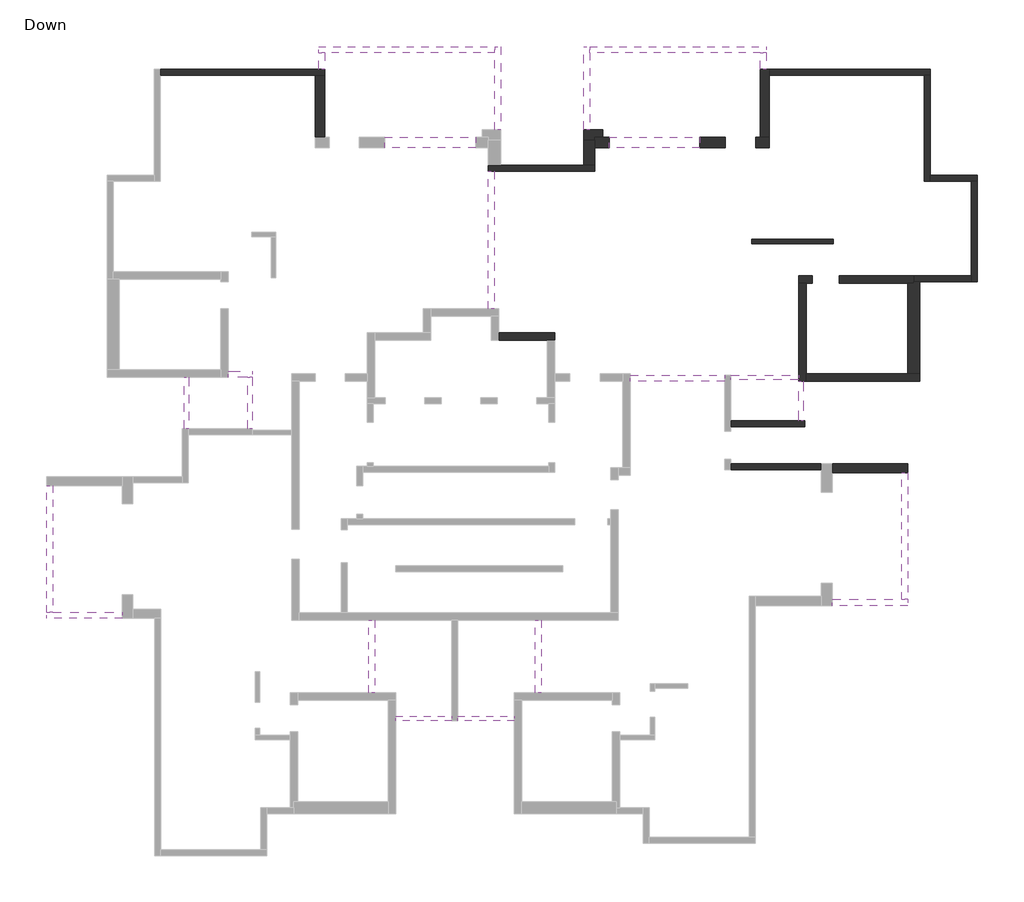
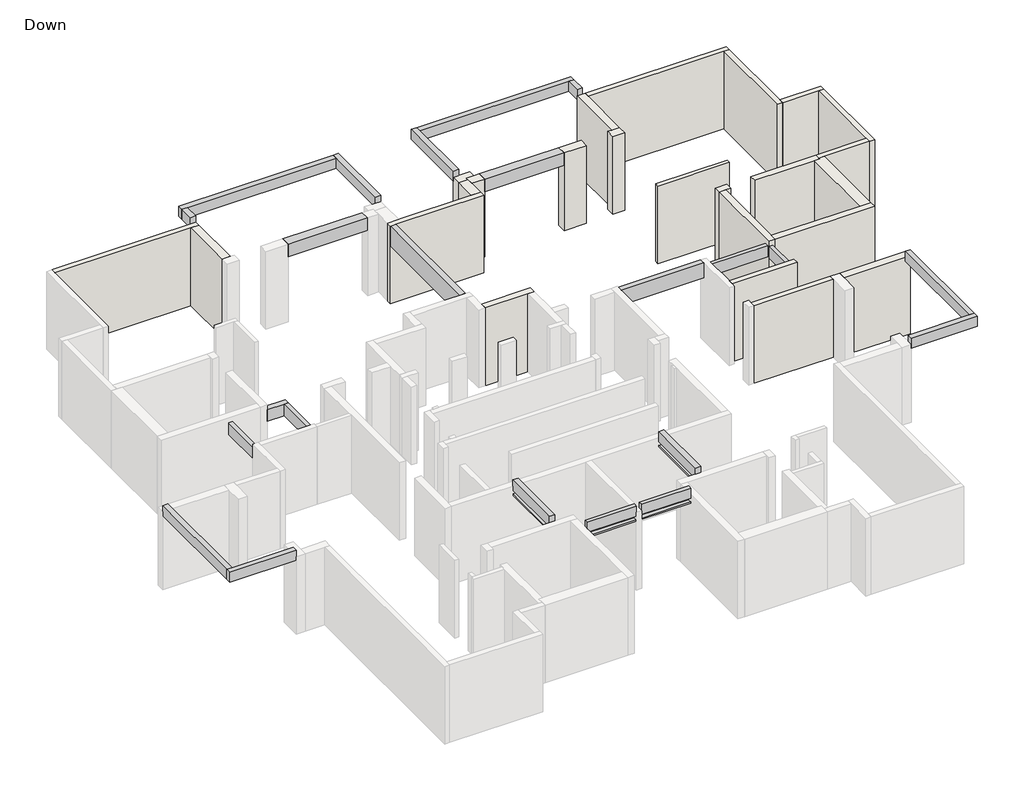
# One storey, part 3 of 3: 24 walls, 23 beams.
"""IFC4 building model written with IfcOpenShell, lengths in millimetres."""

from ifc_helpers import new_model, si_unit, frame, origin, place, context, project, spatial, polyline, outline, extrude, faceted_brep, element, save

model = new_model("IFC4")

# Units and contexts
model_context = context("Model", 3, world=origin())
ifc_project = project(units=[si_unit("LENGTHUNIT", "METRE", prefix="MILLI")], contexts=[model_context])

# Site, building, storey
site = spatial("IfcSite", under=ifc_project)
building = spatial("IfcBuilding", under=site)
storey = spatial("IfcBuildingStorey", under=building, Name="Down", Elevation=0.0)

# Beams
placement = place(None, origin())
element("IfcBeam", 1, ObjectType="Concrete Rectengular Beam : 15/60", at=placement, inside=storey, context=model_context, shape_type="Brep", body=[
    faceted_brep([(26027.850174, -8804.7310591, 2900.0), (26027.850174, -8954.7310591, 2900.0), (26027.850174, -8954.7310591, 2450.0), (26027.850174, -8804.7310591, 2450.0), (26027.850174, -8804.7310591, 2730.0), (23780.6220263, -8954.7310591, 2900.0), (23780.6220263, -8804.7310591, 2900.0), (23780.6220263, -8804.7310591, 2450.0), (23780.6220263, -8954.7310591, 2450.0)], [[[0, 1, 2, 3, 4]], [[5, 6, 7, 8]], [[1, 0, 6, 5]], [[1, 5, 8, 2]], [[6, 0, 4, 3, 7]], [[3, 2, 8, 7]]]),
])
element("IfcBeam", 2, ObjectType="Concrete Rectengular Beam : 15/60", at=placement, inside=storey, context=model_context, shape_type="SweptSolid", body=[
    extrude(outline(polyline([(26177.850174, -10305.7627314), (26027.850174, -10305.7627314), (26027.850174, -9003.4933914), (26177.850174, -9003.4933914), (26177.850174, -10305.7627314)])), frame((0.0, 0.0, 2450.0), z_axis=(0.0, 0.0, 1.0), x_axis=(1.0, 0.0, 0.0)), (0.0, 0.0, 1.0), 450.0),
])
element("IfcBeam", 3, ObjectType="Concrete Rectengular Beam : 15/60", at=placement, inside=storey, context=model_context, shape_type="SweptSolid", body=[
    extrude(outline(polyline([(5696.9503171, -8875.9821525), (5846.9503171, -8875.9821525), (5846.9503171, -10574.5447275), (5696.9503171, -10574.5447275), (5696.9503171, -8875.9821525)])), frame((0.0, 0.0, 2450.0), z_axis=(0.0, 0.0, 1.0), x_axis=(1.0, 0.0, 0.0)), (0.0, 0.0, 1.0), 450.0),
])
element("IfcBeam", 4, ObjectType="Concrete Rectengular Beam : 15/60", at=placement, inside=storey, context=model_context, shape_type="Brep", body=[
    faceted_brep([(7954.0579731, -10574.5447275, 2900.0), (7804.0579731, -10574.5447275, 2900.0), (7804.0579731, -10574.5447275, 2450.0), (7954.0579731, -10574.5447275, 2450.0), (7954.0579731, -10574.5447275, 2730.0), (7954.0579731, -8873.5161743, 2900.0), (7804.0579731, -8873.5161743, 2900.0), (7804.0579731, -8873.5161743, 2450.0), (7954.0579731, -8873.5161743, 2450.0), (7954.0579731, -8873.5161743, 2730.0)], [[[0, 1, 2, 3, 4]], [[1, 0, 5, 6]], [[1, 6, 7, 2]], [[5, 0, 4, 3, 8, 9]], [[6, 5, 9, 8, 7]], [[3, 2, 7, 8]]]),
])
element("IfcBeam", 5, ObjectType="Concrete Rectengular Beam : 15/60", at=placement, inside=storey, context=model_context, shape_type="Brep", body=[
    faceted_brep([(14556.9532328, -20224.3060494, 2750.0), (14556.9532328, -20074.3060494, 2750.0), (14556.9532328, -20074.3060494, 2800.0), (14556.9532328, -20224.3060494, 2800.0), (12702.1320718, -20074.3060494, 2750.0), (12702.1320718, -20224.3060494, 2750.0), (12702.1320718, -20224.3060494, 2800.0), (12702.1320718, -20074.3060494, 2800.0)], [[[0, 1, 2, 3]], [[4, 5, 6, 7]], [[1, 0, 5, 4]], [[1, 4, 7, 2]], [[3, 2, 7, 6]], [[5, 0, 3, 6]]]),
    faceted_brep([(14556.9532328, -20224.3060494, 3350.0), (14556.9532328, -20074.3060494, 3350.0), (12702.1320718, -20074.3060494, 3350.0), (12702.1320718, -20224.3060494, 3350.0), (12702.1320718, -20224.3060494, 2950.0), (14556.9532328, -20224.3060494, 2950.0), (14556.9532328, -20224.3060494, 3100.0), (14556.9532328, -20074.3060494, 2950.0), (12702.1320718, -20074.3060494, 2950.0)], [[[0, 1, 2, 3]], [[0, 3, 4, 5, 6]], [[7, 5, 4, 8]], [[1, 0, 6, 5, 7]], [[3, 2, 8, 4]], [[2, 1, 7, 8]]]),
])
element("IfcBeam", 6, ObjectType="Concrete Rectengular Beam : 15/60", at=placement, inside=storey, context=model_context, shape_type="Brep", body=[
    faceted_brep([(16611.7743938, -20224.3060494, 2750.0), (16611.7743938, -20074.3060494, 2750.0), (16611.7743938, -20074.3060494, 2800.0), (16611.7743938, -20224.3060494, 2800.0), (14756.9532328, -20074.3060494, 2750.0), (14756.9532328, -20224.3060494, 2750.0), (14756.9532328, -20224.3060494, 2800.0), (14756.9532328, -20074.3060494, 2800.0)], [[[0, 1, 2, 3]], [[4, 5, 6, 7]], [[1, 0, 5, 4]], [[1, 4, 7, 2]], [[3, 2, 7, 6]], [[5, 0, 3, 6]]]),
    faceted_brep([(16611.7743938, -20224.3060494, 3350.0), (16611.7743938, -20074.3060494, 3350.0), (14756.9532328, -20074.3060494, 3350.0), (14756.9532328, -20224.3060494, 3350.0), (14756.9532328, -20224.3060494, 3100.0), (14756.9532328, -20224.3060494, 2950.0), (16611.7743938, -20224.3060494, 2950.0), (16611.7743938, -20074.3060494, 2950.0), (14756.9532328, -20074.3060494, 2950.0)], [[[0, 1, 2, 3]], [[0, 3, 4, 5, 6]], [[7, 6, 5, 8]], [[1, 0, 6, 7]], [[3, 2, 8, 5, 4]], [[2, 1, 7, 8]]]),
])
element("IfcBeam", 7, ObjectType="Concrete Rectengular Beam : 20/60", at=placement, inside=storey, context=model_context, shape_type="Brep", body=[
    faceted_brep([(20461.0939579, -8804.7310591, 3100.0), (20461.0939579, -9004.7310591, 3100.0), (23580.6220263, -9004.7310591, 3100.0), (23580.6220263, -8804.7310591, 3100.0), (20461.0939579, -8804.7310591, 2500.0), (20461.0939579, -8804.7310591, 2730.0), (20461.0939579, -8804.7310591, 2950.0), (23580.6220263, -8804.7310591, 2500.0), (20461.0939579, -9004.7310591, 2500.0), (23580.6220263, -9004.7310591, 2500.0), (20461.0939579, -9004.7310591, 2950.0), (20461.0939579, -9004.7310591, 2730.0), (23580.6220263, -9004.7310591, 2730.0), (23580.6220263, -9004.7310591, 2950.0)], [[[0, 1, 2, 3]], [[4, 5, 6, 0, 3, 7]], [[8, 4, 7, 9]], [[1, 10, 11, 8, 9, 12, 13, 2]], [[1, 0, 6, 5, 4, 8, 11, 10]], [[3, 2, 13, 12, 9, 7]]]),
])
element("IfcBeam", 8, ObjectType="Concrete Rectengular Beam : 20/60", at=placement, inside=storey, context=model_context, shape_type="Brep", body=[
    faceted_brep([(16172.9774125, -685.8100602, 3350.0), (15972.9774125, -685.8100602, 3350.0), (15972.9774125, -685.8100602, 2950.0), (16172.9774125, -685.8100602, 2950.0), (16172.9774125, -685.8100602, 3100.0), (16172.9774125, 2066.3547226, 3350.0), (15972.9774125, 2066.3547226, 3350.0), (15972.9774125, 1866.3547226, 3350.0), (16172.9774125, 2066.3547226, 2950.0), (15972.9774125, 2066.3547226, 2950.0), (15972.9774125, 1866.3547226, 2950.0)], [[[0, 1, 2, 3, 4]], [[1, 0, 5, 6, 7]], [[5, 0, 4, 3, 8]], [[1, 7, 6, 9, 10, 2]], [[6, 5, 8, 9]], [[3, 2, 10, 9, 8]]]),
])
element("IfcBeam", 9, ObjectType="Concrete Rectengular Beam : 20/60", at=placement, inside=storey, context=model_context, shape_type="Brep", body=[
    faceted_brep([(10145.0259753, 2066.3547226, 3350.0), (10145.0259753, 1866.3547226, 3350.0), (10345.0259753, 1866.3547226, 3350.0), (15972.9774125, 1866.3547226, 3350.0), (15972.9774125, 2066.3547226, 3350.0), (15972.9774125, 2066.3547226, 2950.0), (10145.0259753, 2066.3547226, 2950.0), (10145.0259753, 1866.3547226, 2950.0), (10345.0259753, 1866.3547226, 2950.0), (15972.9774125, 1866.3547226, 2950.0)], [[[0, 1, 2, 3, 4]], [[0, 4, 5, 6]], [[3, 2, 1, 7, 8, 9]], [[1, 0, 6, 7]], [[4, 3, 9, 5]], [[6, 5, 9, 8, 7]]]),
])
element("IfcBeam", 10, ObjectType="Concrete Rectengular Beam : 20/60", at=placement, inside=storey, context=model_context, shape_type="Brep", body=[
    faceted_brep([(10345.0259753, 1316.3547226, 3350.0), (10145.0259753, 1316.3547226, 3350.0), (10145.0259753, 1316.3547226, 2950.0), (10345.0259753, 1316.3547226, 2950.0), (10345.0259753, 1316.3547226, 3100.0), (10345.0259753, 1866.3547226, 3350.0), (10145.0259753, 1866.3547226, 3350.0), (10145.0259753, 1866.3547226, 2950.0), (10345.0259753, 1866.3547226, 2950.0)], [[[0, 1, 2, 3, 4]], [[1, 0, 5, 6]], [[1, 6, 7, 2]], [[5, 0, 4, 3, 8]], [[6, 5, 8, 7]], [[3, 2, 7, 8]]]),
])
element("IfcBeam", 11, ObjectType="Concrete Rectengular Beam : 20/60", at=placement, inside=storey, context=model_context, shape_type="Brep", body=[
    faceted_brep([(19122.5763384, -685.8100602, 3350.0), (18922.5763384, -685.8100602, 3350.0), (18922.5763384, -685.8100602, 3100.0), (18922.5763384, -685.8100602, 2950.0), (19122.5763384, -685.8100602, 2950.0), (19122.5763384, 1866.3547226, 3350.0), (19122.5763384, 2066.3547226, 3350.0), (18922.5763384, 2066.3547226, 3350.0), (19122.5763384, 1866.3547226, 2950.0), (19122.5763384, 2066.3547226, 2950.0), (18922.5763384, 2066.3547226, 2950.0)], [[[0, 1, 2, 3, 4]], [[1, 0, 5, 6, 7]], [[6, 5, 0, 4, 8, 9]], [[1, 7, 10, 3, 2]], [[7, 6, 9, 10]], [[4, 3, 10, 9, 8]]]),
])
element("IfcBeam", 12, ObjectType="Concrete Rectengular Beam : 20/60", at=placement, inside=storey, context=model_context, shape_type="Brep", body=[
    faceted_brep([(24949.2058247, 1866.3547226, 3350.0), (24949.2058247, 2066.3547226, 3350.0), (19122.5763384, 2066.3547226, 3350.0), (19122.5763384, 1866.3547226, 3350.0), (24749.2058247, 1866.3547226, 3350.0), (19122.5763384, 1866.3547226, 2950.0), (24749.2058247, 1866.3547226, 2950.0), (24949.2058247, 1866.3547226, 2950.0), (24949.2058247, 2066.3547226, 2950.0), (19122.5763384, 2066.3547226, 2950.0)], [[[0, 1, 2, 3, 4]], [[0, 4, 3, 5, 6, 7]], [[2, 1, 8, 9]], [[1, 0, 7, 8]], [[3, 2, 9, 5]], [[7, 6, 5, 9, 8]]]),
])
element("IfcBeam", 13, ObjectType="Concrete Rectengular Beam : 20/60", at=placement, inside=storey, context=model_context, shape_type="Brep", body=[
    faceted_brep([(24949.2058247, 1316.3547226, 3350.0), (24749.2058247, 1316.3547226, 3350.0), (24749.2058247, 1316.3547226, 3100.0), (24749.2058247, 1316.3547226, 2950.0), (24949.2058247, 1316.3547226, 2950.0), (24949.2058247, 1866.3547226, 3350.0), (24749.2058247, 1866.3547226, 3350.0), (24749.2058247, 1866.3547226, 2950.0), (24949.2058247, 1866.3547226, 2950.0)], [[[0, 1, 2, 3, 4]], [[1, 0, 5, 6]], [[1, 6, 7, 3, 2]], [[5, 0, 4, 8]], [[6, 5, 8, 7]], [[4, 3, 7, 8]]]),
])
element("IfcBeam", 14, ObjectType="Concrete Rectengular Beam : 20/60", at=placement, inside=storey, context=model_context, shape_type="Brep", body=[
    faceted_brep([(3654.7368494, -16642.3482114, 3350.0), (3654.7368494, -16842.3482114, 3350.0), (3654.7368494, -16842.3482114, 3100.0), (3654.7368494, -16842.3482114, 2950.0), (3654.7368494, -16642.3482114, 2950.0), (1351.3421966, -16642.3482114, 3350.0), (1151.3421966, -16642.3482114, 3350.0), (1151.3421966, -16842.3482114, 3350.0), (1351.3421966, -16642.3482114, 2950.0), (1151.3421966, -16642.3482114, 2950.0), (1151.3421966, -16842.3482114, 2950.0)], [[[0, 1, 2, 3, 4]], [[1, 0, 5, 6, 7]], [[6, 5, 0, 4, 8, 9]], [[1, 7, 10, 3, 2]], [[7, 6, 9, 10]], [[4, 3, 10, 9, 8]]]),
])
element("IfcBeam", 15, ObjectType="Concrete Rectengular Beam : 20/60", at=placement, inside=storey, context=model_context, shape_type="Brep", body=[
    faceted_brep([(1151.3421966, -12453.0033555, 3350.0), (1351.3421966, -12453.0033555, 3350.0), (1351.3421966, -12453.0033555, 2950.0), (1151.3421966, -12453.0033555, 2950.0), (1151.3421966, -12453.0033555, 3100.0), (1151.3421966, -16642.3482114, 3350.0), (1351.3421966, -16642.3482114, 3350.0), (1351.3421966, -16642.3482114, 2950.0), (1151.3421966, -16642.3482114, 2950.0)], [[[0, 1, 2, 3, 4]], [[1, 0, 5, 6]], [[1, 6, 7, 2]], [[5, 0, 4, 3, 8]], [[6, 5, 8, 7]], [[3, 2, 7, 8]]]),
])
element("IfcBeam", 16, ObjectType="Concrete Rectengular Beam : 20/60", at=placement, inside=storey, context=model_context, shape_type="Brep", body=[
    faceted_brep([(27127.656655, -16418.7263398, 3350.0), (27127.656655, -16218.7263398, 3350.0), (27127.656655, -16218.7263398, 2950.0), (27127.656655, -16418.7263398, 2950.0), (27127.656655, -16418.7263398, 3100.0), (29629.9103996, -16418.7263398, 3350.0), (29629.9103996, -16218.7263398, 3350.0), (29429.9103996, -16218.7263398, 3350.0), (29629.9103996, -16418.7263398, 2950.0), (29629.9103996, -16218.7263398, 2950.0), (29429.9103996, -16218.7263398, 2950.0)], [[[0, 1, 2, 3, 4]], [[1, 0, 5, 6, 7]], [[5, 0, 4, 3, 8]], [[1, 7, 6, 9, 10, 2]], [[6, 5, 8, 9]], [[3, 2, 10, 9, 8]]]),
])
element("IfcBeam", 17, ObjectType="Concrete Rectengular Beam : 20/60", at=placement, inside=storey, context=model_context, shape_type="SweptSolid", body=[
    extrude(outline(polyline([(29429.9103996, -12033.0804512), (29629.9103996, -12033.0804512), (29629.9103996, -16218.7263398), (29429.9103996, -16218.7263398), (29429.9103996, -12033.0804512)])), frame((0.0, 0.0, 2950.0), z_axis=(0.0, 0.0, 1.0), x_axis=(1.0, 0.0, 0.0)), (0.0, 0.0, 1.0), 400.0),
])
element("IfcBeam", 18, ObjectType="Concrete Rectengular Beam : 20/60", at=placement, inside=storey, context=model_context, shape_type="Brep", body=[
    faceted_brep([(7157.9504595, -8873.5161743, 2900.0), (7157.9504595, -8673.5161743, 2900.0), (7157.9504595, -8673.5161743, 2730.0), (7157.9504595, -8673.5161743, 2450.0), (7157.9504595, -8873.5161743, 2450.0), (7804.0579731, -8873.5161743, 2900.0), (7954.0579731, -8873.5161743, 2900.0), (7954.0579731, -8673.5161743, 2900.0), (7804.0579731, -8873.5161743, 2450.0), (7954.0579731, -8873.5161743, 2450.0), (7954.0579731, -8873.5161743, 2730.0), (7954.0579731, -8673.5161743, 2730.0), (7954.0579731, -8673.5161743, 2450.0)], [[[0, 1, 2, 3, 4]], [[1, 0, 5, 6, 7]], [[6, 5, 0, 4, 8, 9, 10]], [[1, 7, 11, 12, 3, 2]], [[7, 6, 10, 9, 12, 11]], [[4, 3, 12, 9, 8]]]),
])
element("IfcBeam", 19, ObjectType="Concrete Rectengular Beam : 20/60", at=placement, inside=storey, context=model_context, shape_type="SweptSolid", body=[
    extrude(outline(polyline([(11800.0437745, -16906.0156488), (12000.0437745, -16906.0156488), (12000.0437745, -19301.9218456), (11800.0437745, -19301.9218456), (11800.0437745, -16906.0156488)])), frame((0.0, 0.0, 2750.0), z_axis=(0.0, 0.0, 1.0), x_axis=(1.0, 0.0, 0.0)), (0.0, 0.0, 1.0), 50.0),
    extrude(outline(polyline([(11800.0437745, -16906.0156488), (12000.0437745, -16906.0156488), (12000.0437745, -19301.9218456), (11800.0437745, -19301.9218456), (11800.0437745, -16906.0156488)])), frame((0.0, 0.0, 2950.0), z_axis=(0.0, 0.0, 1.0), x_axis=(1.0, 0.0, 0.0)), (0.0, 0.0, 1.0), 400.0),
])
element("IfcBeam", 20, ObjectType="Concrete Rectengular Beam : 20/60", at=placement, inside=storey, context=model_context, shape_type="SweptSolid", body=[
    extrude(outline(polyline([(17308.6310988, -16906.0156488), (17508.6310988, -16906.0156488), (17508.6310988, -19301.9218456), (17308.6310988, -19301.9218456), (17308.6310988, -16906.0156488)])), frame((0.0, 0.0, 2750.0), z_axis=(0.0, 0.0, 1.0), x_axis=(1.0, 0.0, 0.0)), (0.0, 0.0, 1.0), 50.0),
    extrude(outline(polyline([(17308.6310988, -16906.0156488), (17508.6310988, -16906.0156488), (17508.6310988, -19301.9218456), (17308.6310988, -19301.9218456), (17308.6310988, -16906.0156488)])), frame((0.0, 0.0, 2950.0), z_axis=(0.0, 0.0, 1.0), x_axis=(1.0, 0.0, 0.0)), (0.0, 0.0, 1.0), 400.0),
])
element("IfcBeam", 21, ObjectType="Concrete Rectengular Beam : 20/80", at=placement, inside=storey, context=model_context, shape_type="Brep", body=[
    faceted_brep([(15755.4299651, -6603.7071845, 3100.0), (15955.4299651, -6603.7071845, 3100.0), (15955.4299651, -2061.9790741, 3100.0), (15755.4299651, -2061.9790741, 3100.0), (15955.4299651, -6603.7071845, 2950.0), (15955.4299651, -6603.7071845, 2730.0), (15955.4299651, -6603.7071845, 2300.0), (15955.4299651, -2061.9790741, 2300.0), (15955.4299651, -2061.9790741, 2730.0), (15955.4299651, -2061.9790741, 2950.0), (15755.4299651, -6603.7071845, 2300.0), (15755.4299651, -2061.9790741, 2300.0), (15755.4299651, -6603.7071845, 2730.0), (15755.4299651, -6603.7071845, 2950.0), (15755.4299651, -2061.9790741, 2950.0), (15755.4299651, -2061.9790741, 2730.0)], [[[0, 1, 2, 3]], [[1, 4, 5, 6, 7, 8, 9, 2]], [[6, 10, 11, 7]], [[10, 12, 13, 0, 3, 14, 15, 11]], [[1, 0, 13, 12, 10, 6, 5, 4]], [[3, 2, 9, 8, 7, 11, 15, 14]]]),
])
element("IfcBeam", 22, ObjectType="Concrete Rectengular Beam : 35/50", at=placement, inside=storey, context=model_context, shape_type="Brep", body=[
    faceted_brep([(12338.469313, -935.8943434, 3100.0), (12338.469313, -1285.8943434, 3100.0), (15339.3043472, -1285.8943434, 3100.0), (15339.3043472, -935.8943434, 3100.0), (12338.469313, -1285.8943434, 2950.0), (12338.469313, -1285.8943434, 2730.0), (12338.469313, -1285.8943434, 2600.0), (15339.3043472, -1285.8943434, 2600.0), (15339.3043472, -1285.8943434, 2730.0), (15339.3043472, -1285.8943434, 2950.0), (12338.469313, -935.8943434, 2600.0), (15339.3043472, -935.8943434, 2600.0), (15339.3043472, -935.8943434, 2950.0), (15339.3043472, -935.8943434, 2730.0), (12338.469313, -935.8943434, 2730.0), (12338.469313, -935.8943434, 2950.0)], [[[0, 1, 2, 3]], [[2, 1, 4, 5, 6, 7, 8, 9]], [[6, 10, 11, 7]], [[0, 3, 12, 13, 11, 10, 14, 15]], [[1, 0, 15, 14, 10, 6, 5, 4]], [[3, 2, 9, 8, 7, 11, 13, 12]]]),
])
element("IfcBeam", 23, ObjectType="Concrete Rectengular Beam : 35/50", at=placement, inside=storey, context=model_context, shape_type="Brep", body=[
    faceted_brep([(19754.9321315, -937.0352516, 3100.0), (19754.9321315, -1287.0352516, 3100.0), (22755.7671656, -1287.0352516, 3100.0), (22755.7671656, -937.0352516, 3100.0), (22755.7671656, -1287.0352516, 2600.0), (22755.7671656, -1287.0352516, 2730.0), (22755.7671656, -1287.0352516, 2950.0), (19754.9321315, -1287.0352516, 2950.0), (19754.9321315, -1287.0352516, 2730.0), (19754.9321315, -1287.0352516, 2600.0), (19754.9321315, -937.0352516, 2600.0), (22755.7671656, -937.0352516, 2600.0), (22755.7671656, -937.0352516, 2950.0), (22755.7671656, -937.0352516, 2730.0), (19754.9321315, -937.0352516, 2730.0), (19754.9321315, -937.0352516, 2950.0)], [[[0, 1, 2, 3]], [[4, 5, 6, 2, 1, 7, 8, 9]], [[9, 10, 11, 4]], [[0, 3, 12, 13, 11, 10, 14, 15]], [[1, 0, 15, 14, 10, 9, 8, 7]], [[3, 2, 6, 5, 4, 11, 13, 12]]]),
])

# Walls
element("IfcWall", 24, ObjectType="15", at=placement, inside=storey, context=model_context, shape_type="Brep", body=[
    faceted_brep([(24469.3206885, -4455.3303309, 0.0), (27166.4567553, -4455.3303309, 0.0), (27166.4567553, -4455.3303309, 2730.0), (27166.4567553, -4455.3303309, 2950.0), (27166.4567553, -4455.3303309, 3100.0), (24469.3206885, -4455.3303309, 3100.0), (24469.3206885, -4455.3303309, 2950.0), (24469.3206885, -4455.3303309, 2730.0), (24469.3206885, -4305.3303309, 0.0), (24469.3206885, -4305.3303309, 2730.0), (24469.3206885, -4305.3303309, 2950.0), (24469.3206885, -4305.3303309, 3100.0), (27166.4567553, -4305.3303309, 3100.0), (27166.4567553, -4305.3303309, 2950.0), (27166.4567553, -4305.3303309, 2730.0), (27166.4567553, -4305.3303309, 0.0)], [[[0, 1, 2, 3, 4, 5, 6, 7]], [[8, 9, 10, 11, 12, 13, 14, 15]], [[1, 0, 8, 15]], [[4, 3, 2, 1, 15, 14, 13, 12]], [[5, 4, 12, 11]], [[0, 7, 6, 5, 11, 10, 9, 8]]]),
])
element("IfcWall", 25, ObjectType="20", at=placement, inside=storey, context=model_context, shape_type="Brep", body=[
    faceted_brep([(4915.8368705, 1116.275118, 0.0), (10045.0259753, 1116.275118, 0.0), (10345.0259753, 1116.275118, 0.0), (10345.0259753, 1116.275118, 3100.0), (10045.0259753, 1116.275118, 3100.0), (4915.8368705, 1116.275118, 3100.0), (4915.8368705, 1116.275118, 2950.0), (4915.8368705, 1116.275118, 2730.0), (4915.8368705, 1316.275118, 0.0), (4915.8368705, 1316.275118, 3100.0), (10345.0259753, 1316.275118, 3100.0), (10345.0259753, 1316.275118, 2950.0), (10345.0259753, 1316.275118, 2730.0), (10345.0259753, 1316.275118, 0.0)], [[[0, 1, 2, 3, 4, 5, 6, 7]], [[8, 9, 10, 11, 12, 13]], [[2, 1, 0, 8, 13]], [[5, 4, 3, 10, 9]], [[0, 7, 6, 5, 9, 8]], [[3, 2, 13, 12, 11, 10]]]),
])
element("IfcWall", 26, ObjectType="20", at=placement, inside=storey, context=model_context, shape_type="Brep", body=[
    faceted_brep([(26777.656655, -11733.0804512, 0.0), (23780.6220263, -11733.0804512, 0.0), (23780.6220263, -11733.0804512, 3100.0), (26777.656655, -11733.0804512, 3100.0), (26777.656655, -11933.0804512, 0.0), (26777.656655, -11933.0804512, 2730.0), (26777.656655, -11933.0804512, 2950.0), (26777.656655, -11933.0804512, 3100.0), (23780.6220263, -11933.0804512, 3100.0), (23780.6220263, -11933.0804512, 0.0)], [[[0, 1, 2, 3]], [[4, 5, 6, 7, 8, 9]], [[1, 0, 4, 9]], [[3, 2, 8, 7]], [[0, 3, 7, 6, 5, 4]], [[2, 1, 9, 8]]]),
])
element("IfcWall", 27, ObjectType="20", at=placement, inside=storey, context=model_context, shape_type="Brep", body=[
    faceted_brep([(23780.6220263, -10505.7627314, 0.0), (26230.3161522, -10505.7627314, 0.0), (26230.3161522, -10505.7627314, 3100.0), (23780.6220263, -10505.7627314, 3100.0), (23780.6220263, -10305.7627314, 0.0), (23780.6220263, -10305.7627314, 2300.0), (23780.6220263, -10305.7627314, 2450.0), (23780.6220263, -10305.7627314, 3100.0), (26230.3161522, -10305.7627314, 3100.0), (26230.3161522, -10305.7627314, 0.0)], [[[0, 1, 2, 3]], [[4, 5, 6, 7, 8, 9]], [[1, 0, 4, 9]], [[2, 1, 9, 8]], [[3, 2, 8, 7]], [[0, 3, 7, 6, 5, 4]]]),
])
element("IfcWall", 28, ObjectType="20", at=placement, inside=storey, context=model_context, shape_type="Brep", body=[
    faceted_brep([(15752.9774125, -2061.9790741, 0.0), (19272.5763384, -2061.9790741, 0.0), (19272.5763384, -2061.9790741, 2730.0), (19272.5763384, -2061.9790741, 2950.0), (19272.5763384, -2061.9790741, 3100.0), (15955.4299651, -2061.9790741, 3100.0), (15755.4299651, -2061.9790741, 3100.0), (15752.9774125, -2061.9790741, 3100.0), (15752.9774125, -2061.9790741, 2950.0), (15752.9774125, -2061.9790741, 2730.0), (15752.9774125, -1861.9790741, 0.0), (15752.9774125, -1861.9790741, 3100.0), (16172.9774125, -1861.9790741, 3100.0), (18922.5763384, -1861.9790741, 3100.0), (19272.5763384, -1861.9790741, 3100.0), (19272.5763384, -1861.9790741, 0.0), (18922.5763384, -1861.9790741, 0.0), (16172.9774125, -1861.9790741, 0.0)], [[[0, 1, 2, 3, 4, 5, 6, 7, 8, 9]], [[10, 11, 12, 13, 14, 15, 16, 17]], [[1, 0, 10, 17, 16, 15]], [[7, 6, 5, 4, 14, 13, 12, 11]], [[4, 3, 2, 1, 15, 14]], [[0, 9, 8, 7, 11, 10]]]),
])
element("IfcWall", 29, ObjectType="20", at=placement, inside=storey, context=model_context, shape_type="Brep", body=[
    faceted_brep([(25049.2058247, 1116.275118, 0.0), (30178.3996082, 1116.275118, 0.0), (30378.3996082, 1116.275118, 0.0), (30378.3996082, 1116.275118, 3100.0), (30178.3996082, 1116.275118, 3100.0), (25049.2058247, 1116.275118, 3100.0), (25049.2058247, 1116.275118, 2950.0), (25049.2058247, 1116.275118, 2730.0), (25049.2058247, 1316.275118, 0.0), (25049.2058247, 1316.275118, 3100.0), (30378.3996082, 1316.275118, 3100.0), (30378.3996082, 1316.275118, 0.0)], [[[0, 1, 2, 3, 4, 5, 6, 7]], [[8, 9, 10, 11]], [[2, 1, 0, 8, 11]], [[5, 4, 3, 10, 9]], [[0, 7, 6, 5, 9, 8]], [[3, 2, 11, 10]]]),
])
element("IfcWall", 30, ObjectType="20", at=placement, inside=storey, context=model_context, shape_type="Brep", body=[
    faceted_brep([(30178.3996082, 1116.275118, 0.0), (30178.3996082, -2383.1380866, 0.0), (30178.3996082, -2383.1380866, 2730.0), (30178.3996082, -2383.1380866, 2950.0), (30178.3996082, -2383.1380866, 3100.0), (30178.3996082, 1116.275118, 3100.0), (30178.3996082, 1116.275118, 2950.0), (30178.3996082, 1116.275118, 2730.0), (30378.3996082, 1116.275118, 0.0), (30378.3996082, 1116.275118, 3100.0), (30378.3996082, -2183.1380866, 3100.0), (30378.3996082, -2383.1380866, 3100.0), (30378.3996082, -2383.1380866, 0.0), (30378.3996082, -2183.1380866, 0.0)], [[[0, 1, 2, 3, 4, 5, 6, 7]], [[8, 9, 10, 11, 12, 13]], [[1, 0, 8, 13, 12]], [[5, 4, 11, 10, 9]], [[0, 7, 6, 5, 9, 8]], [[4, 3, 2, 1, 12, 11]]]),
])
element("IfcWall", 31, ObjectType="20", at=placement, inside=storey, context=model_context, shape_type="Brep", body=[
    faceted_brep([(30378.3996082, -2383.1380866, 0.0), (31735.6945451, -2383.1380866, 0.0), (31935.6945451, -2383.1380866, 0.0), (31935.6945451, -2383.1380866, 3100.0), (31735.6945451, -2383.1380866, 3100.0), (30378.3996082, -2383.1380866, 3100.0), (30378.3996082, -2183.1380866, 0.0), (30378.3996082, -2183.1380866, 3100.0), (31935.6945451, -2183.1380866, 3100.0), (31935.6945451, -2183.1380866, 0.0)], [[[0, 1, 2, 3, 4, 5]], [[6, 7, 8, 9]], [[2, 1, 0, 6, 9]], [[5, 4, 3, 8, 7]], [[0, 5, 7, 6]], [[3, 2, 9, 8]]]),
])
element("IfcWall", 32, ObjectType="20", at=placement, inside=storey, context=model_context, shape_type="Brep", body=[
    faceted_brep([(31735.6945451, -2383.1380866, 0.0), (31735.6945451, -5506.3666818, 0.0), (31735.6945451, -5706.3666818, 0.0), (31735.6945451, -5706.3666818, 3100.0), (31735.6945451, -5506.3666818, 3100.0), (31735.6945451, -2383.1380866, 3100.0), (31735.6945451, -2383.1380866, 2950.0), (31735.6945451, -2383.1380866, 2730.0), (31935.6945451, -2383.1380866, 0.0), (31935.6945451, -2383.1380866, 3100.0), (31935.6945451, -5706.3666818, 3100.0), (31935.6945451, -5706.3666818, 0.0)], [[[0, 1, 2, 3, 4, 5, 6, 7]], [[8, 9, 10, 11]], [[2, 1, 0, 8, 11]], [[5, 4, 3, 10, 9]], [[0, 7, 6, 5, 9, 8]], [[3, 2, 11, 10]]]),
])
element("IfcWall", 33, ObjectType="20", at=placement, inside=storey, context=model_context, shape_type="Brep", body=[
    faceted_brep([(31735.6945451, -5506.3666818, 0.0), (29827.2587, -5506.3666818, 0.0), (29827.2587, -5506.3666818, 3100.0), (31735.6945451, -5506.3666818, 3100.0), (31735.6945451, -5506.3666818, 2950.0), (31735.6945451, -5506.3666818, 2730.0), (31735.6945451, -5706.3666818, 0.0), (31735.6945451, -5706.3666818, 3100.0), (30027.2587, -5706.3666818, 3100.0), (29827.2587, -5706.3666818, 3100.0), (29827.2587, -5706.3666818, 0.0), (30027.2587, -5706.3666818, 0.0)], [[[0, 1, 2, 3, 4, 5]], [[6, 7, 8, 9, 10, 11]], [[1, 0, 6, 11, 10]], [[2, 1, 10, 9]], [[3, 2, 9, 8, 7]], [[0, 5, 4, 3, 7, 6]]]),
])
element("IfcWall", 34, ObjectType="25", at=placement, inside=storey, context=model_context, shape_type="Brep", body=[
    faceted_brep([(16105.4299651, -7653.6026273, 0.0), (17705.1365674, -7653.6026273, 0.0), (17955.1365674, -7653.6026273, 0.0), (17955.1365674, -7653.6026273, 3100.0), (17705.1365674, -7653.6026273, 3100.0), (16105.4299651, -7653.6026273, 3100.0), (16105.4299651, -7403.6026273, 0.0), (16105.4299651, -7403.6026273, 2730.0), (16105.4299651, -7403.6026273, 2950.0), (16105.4299651, -7403.6026273, 3100.0), (17955.1365674, -7403.6026273, 3100.0), (17955.1365674, -7403.6026273, 2950.0), (17955.1365674, -7403.6026273, 2730.0), (17955.1365674, -7403.6026273, 0.0)], [[[0, 1, 2, 3, 4, 5]], [[6, 7, 8, 9, 10, 11, 12, 13]], [[2, 1, 0, 6, 13]], [[5, 4, 3, 10, 9]], [[0, 5, 9, 8, 7, 6]], [[3, 2, 13, 12, 11, 10]]]),
])
element("IfcWall", 35, ObjectType="25", at=placement, inside=storey, context=model_context, shape_type="Brep", body=[
    faceted_brep([(29827.2587, -5506.3666818, 0.0), (27367.2587, -5506.3666818, 0.0), (27367.2587, -5506.3666818, 2730.0), (27367.2587, -5506.3666818, 2950.0), (27367.2587, -5506.3666818, 3100.0), (29827.2587, -5506.3666818, 3100.0), (29827.2587, -5756.3666818, 0.0), (29827.2587, -5756.3666818, 3100.0), (29627.2587, -5756.3666818, 3100.0), (27367.2587, -5756.3666818, 3100.0), (27367.2587, -5756.3666818, 2950.0), (27367.2587, -5756.3666818, 2730.0), (27367.2587, -5756.3666818, 0.0), (29627.2587, -5756.3666818, 0.0), (29827.2587, -5706.3666818, 0.0), (29827.2587, -5706.3666818, 3100.0)], [[[0, 1, 2, 3, 4, 5]], [[6, 7, 8, 9, 10, 11, 12, 13]], [[1, 0, 14, 6, 13, 12]], [[4, 3, 2, 1, 12, 11, 10, 9]], [[5, 4, 9, 8, 7, 15]], [[0, 5, 15, 7, 6, 14]]]),
])
element("IfcWall", 36, ObjectType="25", at=placement, inside=storey, context=model_context, shape_type="Brep", body=[
    faceted_brep([(26467.7022208, -5506.3666818, 0.0), (26027.850174, -5506.3666818, 0.0), (26027.850174, -5506.3666818, 2730.0), (26027.850174, -5506.3666818, 2950.0), (26027.850174, -5506.3666818, 3100.0), (26467.7022208, -5506.3666818, 3100.0), (26467.7022208, -5506.3666818, 2950.0), (26467.7022208, -5506.3666818, 2730.0), (26467.7022208, -5756.3666818, 0.0), (26467.7022208, -5756.3666818, 2730.0), (26467.7022208, -5756.3666818, 2950.0), (26467.7022208, -5756.3666818, 3100.0), (26277.850174, -5756.3666818, 3100.0), (26027.850174, -5756.3666818, 3100.0), (26027.850174, -5756.3666818, 0.0), (26277.850174, -5756.3666818, 0.0)], [[[0, 1, 2, 3, 4, 5, 6, 7]], [[8, 9, 10, 11, 12, 13, 14, 15]], [[1, 0, 8, 15, 14]], [[5, 4, 13, 12, 11]], [[0, 7, 6, 5, 11, 10, 9, 8]], [[4, 3, 2, 1, 14, 13]]]),
])
element("IfcWall", 37, ObjectType="25", at=placement, inside=storey, context=model_context, shape_type="Brep", body=[
    faceted_brep([(26027.850174, -5756.3666818, 0.0), (26027.850174, -9003.4933914, 0.0), (26027.850174, -9003.4933914, 2300.0), (26027.850174, -9003.4933914, 2450.0), (26027.850174, -9003.4933914, 2900.0), (26027.850174, -9003.4933914, 3100.0), (26027.850174, -5756.3666818, 3100.0), (26277.850174, -5756.3666818, 0.0), (26277.850174, -5756.3666818, 2730.0), (26277.850174, -5756.3666818, 2950.0), (26277.850174, -5756.3666818, 3100.0), (26277.850174, -8753.4933914, 3100.0), (26277.850174, -9003.4933914, 3100.0), (26277.850174, -9003.4933914, 0.0), (26277.850174, -8753.4933914, 0.0)], [[[0, 1, 2, 3, 4, 5, 6]], [[7, 8, 9, 10, 11, 12, 13, 14]], [[1, 0, 7, 14, 13]], [[6, 5, 12, 11, 10]], [[0, 6, 10, 9, 8, 7]], [[5, 4, 3, 2, 1, 13, 12]]]),
])
element("IfcWall", 38, ObjectType="25", at=placement, inside=storey, context=model_context, shape_type="Brep", body=[
    faceted_brep([(26277.850174, -9003.4933914, 0.0), (30027.2587, -9003.4933914, 0.0), (30027.2587, -9003.4933914, 3100.0), (26277.850174, -9003.4933914, 3100.0), (26277.850174, -8753.4933914, 0.0), (26277.850174, -8753.4933914, 2730.0), (26277.850174, -8753.4933914, 2950.0), (26277.850174, -8753.4933914, 3100.0), (29627.2587, -8753.4933914, 3100.0), (30027.2587, -8753.4933914, 3100.0), (30027.2587, -8753.4933914, 0.0), (29627.2587, -8753.4933914, 0.0)], [[[0, 1, 2, 3]], [[4, 5, 6, 7, 8, 9, 10, 11]], [[1, 0, 4, 11, 10]], [[3, 2, 9, 8, 7]], [[0, 3, 7, 6, 5, 4]], [[2, 1, 10, 9]]]),
])
element("IfcWall", 39, ObjectType="30", at=placement, inside=storey, context=model_context, shape_type="Brep", body=[
    faceted_brep([(10045.0259753, 1116.275118, 0.0), (10045.0259753, -935.8943434, 0.0), (10045.0259753, -935.8943434, 3100.0), (10045.0259753, 1116.275118, 3100.0), (10045.0259753, 1116.275118, 2950.0), (10045.0259753, 1116.275118, 2730.0), (10345.0259753, 1116.275118, 0.0), (10345.0259753, 1116.275118, 3100.0), (10345.0259753, -935.8943434, 3100.0), (10345.0259753, -935.8943434, 2950.0), (10345.0259753, -935.8943434, 2730.0), (10345.0259753, -935.8943434, 0.0)], [[[0, 1, 2, 3, 4, 5]], [[6, 7, 8, 9, 10, 11]], [[1, 0, 6, 11]], [[3, 2, 8, 7]], [[0, 5, 4, 3, 7, 6]], [[2, 1, 11, 10, 9, 8]]]),
])
element("IfcWall", 40, ObjectType="30", at=placement, inside=storey, context=model_context, shape_type="Brep", body=[
    faceted_brep([(27127.656655, -12033.0804512, 0.0), (29629.9103996, -12033.0804512, 0.0), (29629.9103996, -12033.0804512, 2730.0), (29629.9103996, -12033.0804512, 2950.0), (29629.9103996, -12033.0804512, 3100.0), (27127.656655, -12033.0804512, 3100.0), (27127.656655, -12033.0804512, 2950.0), (27127.656655, -12033.0804512, 2730.0), (27127.656655, -11733.0804512, 0.0), (27127.656655, -11733.0804512, 3100.0), (29629.9103996, -11733.0804512, 3100.0), (29629.9103996, -11733.0804512, 0.0)], [[[0, 1, 2, 3, 4, 5, 6, 7]], [[8, 9, 10, 11]], [[1, 0, 8, 11]], [[4, 3, 2, 1, 11, 10]], [[5, 4, 10, 9]], [[0, 7, 6, 5, 9, 8]]]),
])
element("IfcWall", 41, ObjectType="30", at=placement, inside=storey, context=model_context, shape_type="Brep", body=[
    faceted_brep([(25049.2058247, -937.0352516, 0.0), (25049.2058247, 1116.275118, 0.0), (25049.2058247, 1316.275118, 0.0), (25049.2058247, 1316.275118, 3100.0), (25049.2058247, 1116.275118, 3100.0), (25049.2058247, -937.0352516, 3100.0), (24749.2058247, -937.0352516, 0.0), (24749.2058247, -937.0352516, 2730.0), (24749.2058247, -937.0352516, 2950.0), (24749.2058247, -937.0352516, 3100.0), (24749.2058247, 1316.275118, 3100.0), (24749.2058247, 1316.275118, 2950.0), (24749.2058247, 1316.275118, 2730.0), (24749.2058247, 1316.275118, 0.0)], [[[0, 1, 2, 3, 4, 5]], [[6, 7, 8, 9, 10, 11, 12, 13]], [[2, 1, 0, 6, 13]], [[5, 4, 3, 10, 9]], [[0, 5, 9, 8, 7, 6]], [[3, 2, 13, 12, 11, 10]]]),
])
element("IfcWall", 42, ObjectType="35", at=placement, inside=storey, context=model_context, shape_type="Brep", body=[
    faceted_brep([(19272.5763384, -1861.9790741, 0.0), (19272.5763384, -1287.0352516, 0.0), (19272.5763384, -1035.8100602, 0.0), (19272.5763384, -1035.8100602, 3100.0), (19272.5763384, -1287.0352516, 3100.0), (19272.5763384, -1861.9790741, 3100.0), (18922.5763384, -1861.9790741, 0.0), (18922.5763384, -1861.9790741, 3100.0), (18922.5763384, -1035.8100602, 3100.0), (18922.5763384, -1035.8100602, 0.0)], [[[0, 1, 2, 3, 4, 5]], [[6, 7, 8, 9]], [[2, 1, 0, 6, 9]], [[5, 4, 3, 8, 7]], [[0, 5, 7, 6]], [[3, 2, 9, 8]]]),
])
element("IfcWall", 43, ObjectType="35", at=placement, inside=storey, context=model_context, shape_type="Brep", body=[
    faceted_brep([(19754.9321315, -937.0352516, 0.0), (19547.5279587, -937.0352516, 0.0), (19272.5763384, -937.0352516, 0.0), (19272.5763384, -937.0352516, 3100.0), (19547.5279587, -937.0352516, 3100.0), (19754.9321315, -937.0352516, 3100.0), (19754.9321315, -937.0352516, 2600.0), (19754.9321315, -1287.0352516, 0.0), (19754.9321315, -1287.0352516, 2600.0), (19754.9321315, -1287.0352516, 3100.0), (19272.5763384, -1287.0352516, 3100.0), (19272.5763384, -1287.0352516, 2950.0), (19272.5763384, -1287.0352516, 2730.0), (19272.5763384, -1287.0352516, 0.0), (19272.5763384, -1035.8100602, 0.0), (19272.5763384, -1035.8100602, 3100.0)], [[[0, 1, 2, 3, 4, 5, 6]], [[7, 8, 9, 10, 11, 12, 13]], [[2, 1, 0, 7, 13, 14]], [[5, 4, 3, 15, 10, 9]], [[0, 6, 5, 9, 8, 7]], [[3, 2, 14, 13, 12, 11, 10, 15]]]),
])
element("IfcWall", 44, ObjectType="35", at=placement, inside=storey, context=model_context, shape_type="Brep", body=[
    faceted_brep([(22755.7671656, -1287.0352516, 0.0), (23598.2584356, -1287.0352516, 0.0), (23598.2584356, -1287.0352516, 2730.0), (23598.2584356, -1287.0352516, 2950.0), (23598.2584356, -1287.0352516, 3100.0), (22755.7671656, -1287.0352516, 3100.0), (22755.7671656, -1287.0352516, 2600.0), (22755.7671656, -937.0352516, 0.0), (22755.7671656, -937.0352516, 2600.0), (22755.7671656, -937.0352516, 3100.0), (23598.2584356, -937.0352516, 3100.0), (23598.2584356, -937.0352516, 2950.0), (23598.2584356, -937.0352516, 2730.0), (23598.2584356, -937.0352516, 0.0)], [[[0, 1, 2, 3, 4, 5, 6]], [[7, 8, 9, 10, 11, 12, 13]], [[1, 0, 7, 13]], [[4, 3, 2, 1, 13, 12, 11, 10]], [[5, 4, 10, 9]], [[0, 6, 5, 9, 8, 7]]]),
])
element("IfcWall", 45, ObjectType="35", at=placement, inside=storey, context=model_context, shape_type="Brep", body=[
    faceted_brep([(25049.2058247, -937.0352516, 0.0), (24749.2058247, -937.0352516, 0.0), (24600.5355733, -937.0352516, 0.0), (24600.5355733, -937.0352516, 2730.0), (24600.5355733, -937.0352516, 2950.0), (24600.5355733, -937.0352516, 3100.0), (24749.2058247, -937.0352516, 3100.0), (25049.2058247, -937.0352516, 3100.0), (25049.2058247, -1287.0352516, 0.0), (25049.2058247, -1287.0352516, 2730.0), (25049.2058247, -1287.0352516, 2950.0), (25049.2058247, -1287.0352516, 3100.0), (24600.5355733, -1287.0352516, 3100.0), (24600.5355733, -1287.0352516, 2950.0), (24600.5355733, -1287.0352516, 2730.0), (24600.5355733, -1287.0352516, 0.0)], [[[0, 1, 2, 3, 4, 5, 6, 7]], [[8, 9, 10, 11, 12, 13, 14, 15]], [[2, 1, 0, 8, 15]], [[5, 4, 3, 2, 15, 14, 13, 12]], [[7, 6, 5, 12, 11]], [[0, 7, 11, 10, 9, 8]]]),
])
element("IfcWall", 46, ObjectType="35", at=placement, inside=storey, context=model_context, shape_type="Brep", body=[
    faceted_brep([(19547.5279587, -685.8100602, 0.0), (18922.5763384, -685.8100602, 0.0), (18922.5763384, -685.8100602, 2730.0), (18922.5763384, -685.8100602, 2950.0), (18922.5763384, -685.8100602, 3100.0), (19547.5279587, -685.8100602, 3100.0), (19547.5279587, -685.8100602, 2950.0), (19547.5279587, -685.8100602, 2730.0), (18922.5763384, -1035.8100602, 3100.0), (18922.5763384, -1035.8100602, 0.0), (19272.5763384, -1035.8100602, 0.0), (19272.5763384, -1035.8100602, 3100.0), (19547.5279587, -937.0352516, 0.0), (19272.5763384, -937.0352516, 0.0), (19272.5763384, -937.0352516, 3100.0), (19547.5279587, -937.0352516, 3100.0), (19547.5279587, -937.0352516, 2950.0), (19547.5279587, -937.0352516, 2730.0)], [[[0, 1, 2, 3, 4, 5, 6, 7]], [[8, 9, 10, 11]], [[1, 0, 12, 13, 10, 9]], [[5, 4, 8, 11, 14, 15]], [[0, 7, 6, 5, 15, 16, 17, 12]], [[4, 3, 2, 1, 9, 8]], [[14, 13, 12, 17, 16, 15]], [[13, 14, 11, 10]]]),
])
element("IfcWall", 47, ObjectType="40", at=placement, inside=storey, context=model_context, shape_type="Brep", body=[
    faceted_brep([(30027.2587, -8753.4933914, 0.0), (30027.2587, -5706.3666818, 0.0), (30027.2587, -5706.3666818, 3100.0), (30027.2587, -8753.4933914, 3100.0), (29627.2587, -8753.4933914, 0.0), (29627.2587, -8753.4933914, 2730.0), (29627.2587, -8753.4933914, 2950.0), (29627.2587, -8753.4933914, 3100.0), (29627.2587, -5756.3666818, 3100.0), (29627.2587, -5756.3666818, 2950.0), (29627.2587, -5756.3666818, 2730.0), (29627.2587, -5756.3666818, 0.0), (29827.2587, -5756.3666818, 0.0), (29827.2587, -5706.3666818, 0.0), (29827.2587, -5706.3666818, 3100.0), (29827.2587, -5756.3666818, 3100.0)], [[[0, 1, 2, 3]], [[4, 5, 6, 7, 8, 9, 10, 11]], [[1, 0, 4, 11, 12, 13]], [[3, 2, 14, 15, 8, 7]], [[2, 1, 13, 14]], [[13, 12, 15, 14]], [[12, 11, 10, 9, 8, 15]], [[0, 3, 7, 6, 5, 4]]]),
])

save(model, "model.ifc")

# Revit data of these elements
# Type "Concrete Rectengular Beam : 15/60"
#   Length [instance default] = 152.4 cm
#   b = 15 cm
#   h = 60 cm
#   Structural Material [instance default] = Concrete
#   Assembly Code = ""
# Type "Concrete Rectengular Beam : 20/60"
#   Length [instance default] = 152.4 cm
#   b = 20 cm
#   h = 60 cm
#   Structural Material [instance default] = Concrete
#   Assembly Code = ""
# Type "Concrete Rectengular Beam : 20/80"
#   Length [instance default] = 152.4 cm
#   b = 20 cm
#   h = 80 cm
#   Structural Material [instance default] = Concrete
#   Assembly Code = ""
# Type "Concrete Rectengular Beam : 35/50"
#   Length [instance default] = 152.4 cm
#   b = 35 cm
#   h = 50 cm
#   Structural Material [instance default] = Concrete
#   Assembly Code = ""
# Type "15"
#   Layers, outside or top first: 15 cm "Concrete" (function 1)
# Type "20"
#   Layers, outside or top first: 20 cm "Concrete" (function 1)
# Type "25"
#   Layers, outside or top first: 25 cm "Concrete" (function 1)
# Type "30"
#   Layers, outside or top first: 30 cm "Concrete" (function 1)
# Type "35"
#   Layers, outside or top first: 35 cm "Concrete" (function 1)
# Type "40"
#   Layers, outside or top first: 40 cm "Concrete" (function 1)
# Element 1 (IfcBeam, "Concrete Rectengular Beam : 15/60")
#   Comments = ""
#   Mark = "B1"
#   SOFiSTiK_AMG_Comments = ""
#   SOFiSTiK_AMG_Scheduled = yes
#   SOFiSTiK_AMG_Adjusted = yes
#   Structural Material = Concrete
#   Phase Created = New Construction
#   Materials on its faces: "Concrete"
# Element 2 (IfcBeam, "Concrete Rectengular Beam : 15/60")
#   Comments = ""
#   Mark = "B2"
#   SOFiSTiK_AMG_Comments = ""
#   SOFiSTiK_AMG_Scheduled = yes
#   SOFiSTiK_AMG_Adjusted = yes
#   Structural Material = Concrete
#   Phase Created = New Construction
#   Materials on its faces: "Concrete"
# Element 3 (IfcBeam, "Concrete Rectengular Beam : 15/60")
#   Comments = ""
#   Mark = "B3"
#   SOFiSTiK_AMG_Comments = ""
#   SOFiSTiK_AMG_Scheduled = yes
#   SOFiSTiK_AMG_Adjusted = yes
#   Structural Material = Concrete
#   Phase Created = New Construction
#   Materials on its faces: "Concrete"
# Element 4 (IfcBeam, "Concrete Rectengular Beam : 15/60")
#   Comments = ""
#   Mark = "B4"
#   SOFiSTiK_AMG_Comments = ""
#   SOFiSTiK_AMG_Scheduled = yes
#   SOFiSTiK_AMG_Adjusted = yes
#   Structural Material = Concrete
#   Phase Created = New Construction
#   Materials on its faces: "Concrete"
# Element 5 (IfcBeam, "Concrete Rectengular Beam : 15/60")
#   Comments = ""
#   Mark = "B5"
#   SOFiSTiK_AMG_Comments = ""
#   SOFiSTiK_AMG_Scheduled = yes
#   SOFiSTiK_AMG_Adjusted = yes
#   Structural Material = Concrete
#   Phase Created = New Construction
#   Materials on its faces: "Concrete"
# Element 6 (IfcBeam, "Concrete Rectengular Beam : 15/60")
#   Comments = ""
#   Mark = "B6"
#   SOFiSTiK_AMG_Comments = ""
#   SOFiSTiK_AMG_Scheduled = yes
#   SOFiSTiK_AMG_Adjusted = yes
#   Structural Material = Concrete
#   Phase Created = New Construction
#   Materials on its faces: "Concrete"
# Element 7 (IfcBeam, "Concrete Rectengular Beam : 20/60")
#   Comments = ""
#   Mark = "B8"
#   SOFiSTiK_AMG_Comments = ""
#   SOFiSTiK_AMG_Scheduled = yes
#   SOFiSTiK_AMG_Adjusted = yes
#   Structural Material = Concrete
#   Phase Created = New Construction
#   Materials on its faces: "Concrete"
# Element 8 (IfcBeam, "Concrete Rectengular Beam : 20/60")
#   Comments = ""
#   Mark = "B9"
#   SOFiSTiK_AMG_Comments = ""
#   SOFiSTiK_AMG_Scheduled = yes
#   SOFiSTiK_AMG_Adjusted = yes
#   Structural Material = Concrete
#   Phase Created = New Construction
#   Materials on its faces: "Concrete"
# Element 9 (IfcBeam, "Concrete Rectengular Beam : 20/60")
#   Comments = ""
#   Mark = "B10"
#   SOFiSTiK_AMG_Comments = ""
#   SOFiSTiK_AMG_Scheduled = yes
#   SOFiSTiK_AMG_Adjusted = yes
#   Structural Material = Concrete
#   Phase Created = New Construction
#   Materials on its faces: "Concrete"
# Element 10 (IfcBeam, "Concrete Rectengular Beam : 20/60")
#   Comments = ""
#   Mark = "B11"
#   SOFiSTiK_AMG_Comments = ""
#   SOFiSTiK_AMG_Scheduled = yes
#   SOFiSTiK_AMG_Adjusted = yes
#   Structural Material = Concrete
#   Phase Created = New Construction
#   Materials on its faces: "Concrete"
# Element 11 (IfcBeam, "Concrete Rectengular Beam : 20/60")
#   Comments = ""
#   Mark = "B12"
#   SOFiSTiK_AMG_Comments = ""
#   SOFiSTiK_AMG_Scheduled = yes
#   SOFiSTiK_AMG_Adjusted = yes
#   Structural Material = Concrete
#   Phase Created = New Construction
#   Materials on its faces: "Concrete"
# Element 12 (IfcBeam, "Concrete Rectengular Beam : 20/60")
#   Comments = ""
#   Mark = "B13"
#   SOFiSTiK_AMG_Comments = ""
#   SOFiSTiK_AMG_Scheduled = yes
#   SOFiSTiK_AMG_Adjusted = yes
#   Structural Material = Concrete
#   Phase Created = New Construction
#   Materials on its faces: "Concrete"
# Element 13 (IfcBeam, "Concrete Rectengular Beam : 20/60")
#   Comments = ""
#   Mark = "B14"
#   SOFiSTiK_AMG_Comments = ""
#   SOFiSTiK_AMG_Scheduled = yes
#   SOFiSTiK_AMG_Adjusted = yes
#   Structural Material = Concrete
#   Phase Created = New Construction
#   Materials on its faces: "Concrete"
# Element 14 (IfcBeam, "Concrete Rectengular Beam : 20/60")
#   Comments = ""
#   Mark = "B15"
#   SOFiSTiK_AMG_Comments = ""
#   SOFiSTiK_AMG_Scheduled = yes
#   SOFiSTiK_AMG_Adjusted = yes
#   Structural Material = Concrete
#   Phase Created = New Construction
#   Materials on its faces: "Concrete"
# Element 15 (IfcBeam, "Concrete Rectengular Beam : 20/60")
#   Comments = ""
#   Mark = "B16"
#   SOFiSTiK_AMG_Comments = ""
#   SOFiSTiK_AMG_Scheduled = yes
#   SOFiSTiK_AMG_Adjusted = yes
#   Structural Material = Concrete
#   Phase Created = New Construction
#   Materials on its faces: "Concrete"
# Element 16 (IfcBeam, "Concrete Rectengular Beam : 20/60")
#   Comments = ""
#   Mark = "B17"
#   SOFiSTiK_AMG_Comments = ""
#   SOFiSTiK_AMG_Scheduled = yes
#   SOFiSTiK_AMG_Adjusted = yes
#   Structural Material = Concrete
#   Phase Created = New Construction
#   Materials on its faces: "Concrete"
# Element 17 (IfcBeam, "Concrete Rectengular Beam : 20/60")
#   Comments = ""
#   Mark = "B18"
#   SOFiSTiK_AMG_Comments = ""
#   SOFiSTiK_AMG_Scheduled = yes
#   SOFiSTiK_AMG_Adjusted = yes
#   Structural Material = Concrete
#   Phase Created = New Construction
#   Materials on its faces: "Concrete"
# Element 18 (IfcBeam, "Concrete Rectengular Beam : 20/60")
#   Comments = ""
#   Mark = "B19"
#   SOFiSTiK_AMG_Comments = ""
#   SOFiSTiK_AMG_Scheduled = yes
#   SOFiSTiK_AMG_Adjusted = yes
#   Structural Material = Concrete
#   Phase Created = New Construction
#   Materials on its faces: "Concrete"
# Element 19 (IfcBeam, "Concrete Rectengular Beam : 20/60")
#   Comments = ""
#   Mark = "B20"
#   SOFiSTiK_AMG_Comments = ""
#   SOFiSTiK_AMG_Scheduled = yes
#   SOFiSTiK_AMG_Adjusted = yes
#   Structural Material = Concrete
#   Phase Created = New Construction
#   Materials on its faces: "Concrete"
# Element 20 (IfcBeam, "Concrete Rectengular Beam : 20/60")
#   Comments = ""
#   Mark = "B21"
#   SOFiSTiK_AMG_Comments = ""
#   SOFiSTiK_AMG_Scheduled = yes
#   SOFiSTiK_AMG_Adjusted = yes
#   Structural Material = Concrete
#   Phase Created = New Construction
#   Materials on its faces: "Concrete"
# Element 21 (IfcBeam, "Concrete Rectengular Beam : 20/80")
#   Comments = ""
#   Mark = "B22"
#   SOFiSTiK_AMG_Comments = ""
#   SOFiSTiK_AMG_Scheduled = yes
#   SOFiSTiK_AMG_Adjusted = yes
#   Structural Material = Concrete
#   Phase Created = New Construction
#   Materials on its faces: "Concrete"
# Element 22 (IfcBeam, "Concrete Rectengular Beam : 35/50")
#   Comments = ""
#   Mark = "B23"
#   SOFiSTiK_AMG_Comments = ""
#   SOFiSTiK_AMG_Scheduled = yes
#   SOFiSTiK_AMG_Adjusted = yes
#   Structural Material = Concrete
#   Phase Created = New Construction
#   Materials on its faces: "Concrete"
# Element 23 (IfcBeam, "Concrete Rectengular Beam : 35/50")
#   Comments = ""
#   Mark = "B24"
#   SOFiSTiK_AMG_Comments = ""
#   SOFiSTiK_AMG_Scheduled = yes
#   SOFiSTiK_AMG_Adjusted = yes
#   Structural Material = Concrete
#   Phase Created = New Construction
#   Materials on its faces: "Concrete"
# Element 24 (IfcWall, "15")
#   Comments = ""
#   Mark = "W108"
#   SOFiSTiK_EdgeZones = "W112"
#   SOFiSTiK_AMG_Comments = ""
#   Top Offset = 0 cm
#   Base Offset = 0 cm
#   wall height = 310 cm
#   SOFiSTiK_AMG_Scheduled = yes
#   SOFiSTiK_AMG_Adjusted = yes
#   Phase Created = New Construction
#   Base Constraint = Down
#   Top Constraint = Typical Floor
#   Materials on its faces: "Concrete"
# Element 25 (IfcWall, "20")
#   Comments = ""
#   Mark = "W4"
#   SOFiSTiK_EdgeZones = "W4"
#   SOFiSTiK_AMG_Comments = ""
#   Top Offset = 0 cm
#   Base Offset = 0 cm
#   wall height = 310 cm
#   SOFiSTiK_AMG_Scheduled = yes
#   SOFiSTiK_AMG_Adjusted = yes
#   Phase Created = New Construction
#   Base Constraint = Down
#   Top Constraint = Typical Floor
#   Materials on its faces: "Concrete"
# Element 26 (IfcWall, "20")
#   Comments = ""
#   Mark = "W17"
#   SOFiSTiK_EdgeZones = "W17"
#   SOFiSTiK_AMG_Comments = ""
#   Top Offset = 0 cm
#   Base Offset = 0 cm
#   wall height = 310 cm
#   SOFiSTiK_AMG_Scheduled = yes
#   SOFiSTiK_AMG_Adjusted = yes
#   Phase Created = New Construction
#   Base Constraint = Down
#   Top Constraint = Typical Floor
#   Materials on its faces: "Concrete"
# Element 27 (IfcWall, "20")
#   Comments = ""
#   Mark = "W20"
#   SOFiSTiK_EdgeZones = "W20"
#   SOFiSTiK_AMG_Comments = ""
#   Top Offset = 0 cm
#   Base Offset = 0 cm
#   wall height = 310 cm
#   SOFiSTiK_AMG_Scheduled = yes
#   SOFiSTiK_AMG_Adjusted = yes
#   Phase Created = New Construction
#   Base Constraint = Down
#   Top Constraint = Typical Floor
#   Materials on its faces: "Concrete"
# Element 28 (IfcWall, "20")
#   Comments = ""
#   Mark = "W21"
#   SOFiSTiK_EdgeZones = "W21"
#   SOFiSTiK_AMG_Comments = ""
#   Top Offset = 0 cm
#   Base Offset = 0 cm
#   wall height = 310 cm
#   SOFiSTiK_AMG_Scheduled = yes
#   SOFiSTiK_AMG_Adjusted = yes
#   Phase Created = New Construction
#   Base Constraint = Down
#   Top Constraint = Typical Floor
#   Materials on its faces: "Concrete"
# Element 29 (IfcWall, "20")
#   Comments = ""
#   Mark = "W22"
#   SOFiSTiK_EdgeZones = "W22"
#   SOFiSTiK_AMG_Comments = ""
#   Top Offset = 0 cm
#   Base Offset = 0 cm
#   wall height = 310 cm
#   SOFiSTiK_AMG_Scheduled = yes
#   SOFiSTiK_AMG_Adjusted = yes
#   Phase Created = New Construction
#   Base Constraint = Down
#   Top Constraint = Typical Floor
#   Materials on its faces: "Concrete"
# Element 30 (IfcWall, "20")
#   Comments = ""
#   Mark = "W23"
#   SOFiSTiK_EdgeZones = "W23"
#   SOFiSTiK_AMG_Comments = ""
#   Top Offset = 0 cm
#   Base Offset = 0 cm
#   wall height = 310 cm
#   SOFiSTiK_AMG_Scheduled = yes
#   SOFiSTiK_AMG_Adjusted = yes
#   Phase Created = New Construction
#   Base Constraint = Down
#   Top Constraint = Typical Floor
#   Materials on its faces: "Concrete"
# Element 31 (IfcWall, "20")
#   Comments = ""
#   Mark = "W24"
#   SOFiSTiK_EdgeZones = "W24"
#   SOFiSTiK_AMG_Comments = ""
#   Top Offset = 0 cm
#   Base Offset = 0 cm
#   wall height = 310 cm
#   SOFiSTiK_AMG_Scheduled = yes
#   SOFiSTiK_AMG_Adjusted = yes
#   Phase Created = New Construction
#   Base Constraint = Down
#   Top Constraint = Typical Floor
#   Materials on its faces: "Concrete"
# Element 32 (IfcWall, "20")
#   Comments = ""
#   Mark = "W25"
#   SOFiSTiK_EdgeZones = "W25"
#   SOFiSTiK_AMG_Comments = ""
#   Top Offset = 0 cm
#   Base Offset = 0 cm
#   wall height = 310 cm
#   SOFiSTiK_AMG_Scheduled = yes
#   SOFiSTiK_AMG_Adjusted = yes
#   Phase Created = New Construction
#   Base Constraint = Down
#   Top Constraint = Typical Floor
#   Materials on its faces: "Concrete"
# Element 33 (IfcWall, "20")
#   Comments = ""
#   Mark = "W26"
#   SOFiSTiK_EdgeZones = "W26"
#   SOFiSTiK_AMG_Comments = ""
#   Top Offset = 0 cm
#   Base Offset = 0 cm
#   wall height = 310 cm
#   SOFiSTiK_AMG_Scheduled = yes
#   SOFiSTiK_AMG_Adjusted = yes
#   Phase Created = New Construction
#   Base Constraint = Down
#   Top Constraint = Typical Floor
#   Materials on its faces: "Concrete"
# Element 34 (IfcWall, "25")
#   Comments = ""
#   Mark = "W90"
#   SOFiSTiK_EdgeZones = "W94"
#   SOFiSTiK_AMG_Comments = ""
#   Top Offset = 0 cm
#   Base Offset = 0 cm
#   wall height = 310 cm
#   SOFiSTiK_AMG_Scheduled = yes
#   SOFiSTiK_AMG_Adjusted = yes
#   Phase Created = New Construction
#   Base Constraint = Down
#   Top Constraint = Typical Floor
#   Materials on its faces: "Concrete"
# Element 35 (IfcWall, "25")
#   Comments = ""
#   Mark = "W92"
#   SOFiSTiK_EdgeZones = "W96"
#   SOFiSTiK_AMG_Comments = ""
#   Top Offset = 0 cm
#   Base Offset = 0 cm
#   wall height = 310 cm
#   SOFiSTiK_AMG_Scheduled = yes
#   SOFiSTiK_AMG_Adjusted = yes
#   Phase Created = New Construction
#   Base Constraint = Down
#   Top Constraint = Typical Floor
#   Materials on its faces: "Concrete"
# Element 36 (IfcWall, "25")
#   Comments = ""
#   Mark = "W93"
#   SOFiSTiK_EdgeZones = "W97"
#   SOFiSTiK_AMG_Comments = ""
#   Top Offset = 0 cm
#   Base Offset = 0 cm
#   wall height = 310 cm
#   SOFiSTiK_AMG_Scheduled = yes
#   SOFiSTiK_AMG_Adjusted = yes
#   Phase Created = New Construction
#   Base Constraint = Down
#   Top Constraint = Typical Floor
#   Materials on its faces: "Concrete"
# Element 37 (IfcWall, "25")
#   Comments = ""
#   Mark = "W94"
#   SOFiSTiK_EdgeZones = "W98"
#   SOFiSTiK_AMG_Comments = ""
#   Top Offset = 0 cm
#   Base Offset = 0 cm
#   wall height = 310 cm
#   SOFiSTiK_AMG_Scheduled = yes
#   SOFiSTiK_AMG_Adjusted = yes
#   Phase Created = New Construction
#   Base Constraint = Down
#   Top Constraint = Typical Floor
#   Materials on its faces: "Concrete"
# Element 38 (IfcWall, "25")
#   Comments = ""
#   Mark = "W95"
#   SOFiSTiK_EdgeZones = "W99"
#   SOFiSTiK_AMG_Comments = ""
